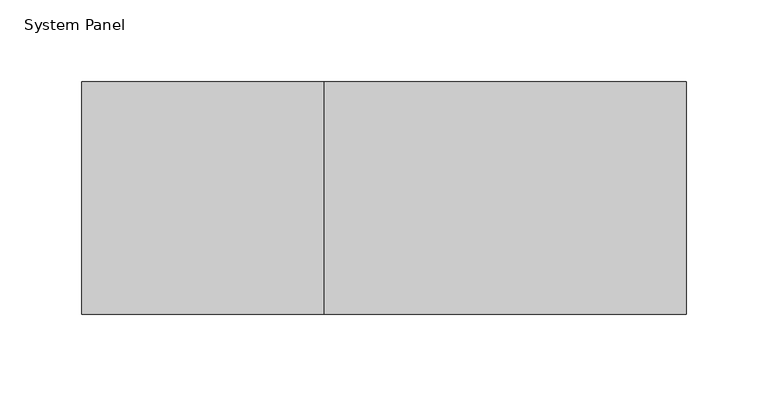
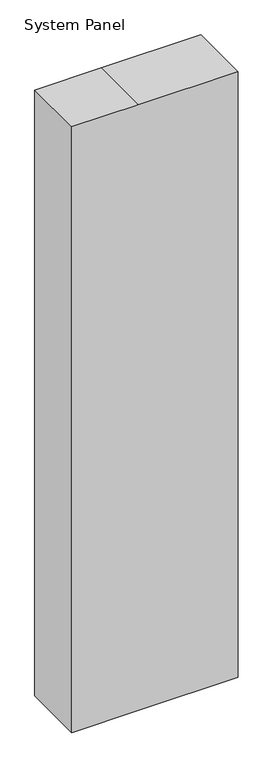
"""IFC4 building model written with IfcOpenShell, lengths in millimetres: plate geometry, System Panel : NLRS_21_CWP_hsb-vulling minerale wol 142 _gen_rsf."""

from ifc_helpers import new_model, si_unit, frame, origin, place, context, project, spatial, polyline, outline, extrude, source, transform, mapped, element, save


def system_panel_d55a1cbf(model_context):
    return source(origin(), model_context, "Body", "SweptSolid", [
        extrude(outline(polyline([(0.0, -184.5), (0.0, -36.3441061), (0.0, 184.5), (1421.0, 184.5), (1421.0, -36.3441061), (1421.0, -184.5), (0.0, -184.5)])), frame((0.0, -71.0, 0.0), z_axis=(0.0, 1.0, 0.0), x_axis=(0.0, 0.0, 1.0)), (0.0, 0.0, 1.0), 142.0),
    ])


if __name__ == "__main__":
    model = new_model("IFC4")
    model_context = context("Model", 3, world=origin())
    ifc_project = project(units=[si_unit("LENGTHUNIT", "METRE", prefix="MILLI")], contexts=[model_context])
    site = spatial("IfcSite", under=ifc_project)
    building = spatial("IfcBuilding", under=site)
    placement = place(None, origin())
    system_panel_shape = system_panel_d55a1cbf(model_context)
    element("IfcPlate", 1, ObjectType="System Panel : NLRS_21_CWP_hsb-vulling minerale wol 142 _gen_rsf", at=placement, inside=building, context=model_context, shape_type="MappedRepresentation", body=[
        mapped(system_panel_shape, transform((0.0, 0.0, 0.0), x_axis=(1.0, 0.0, 0.0), y_axis=(0.0, 1.0, 0.0), z_axis=(0.0, 0.0, 1.0))),
    ])
    save(model, "model.ifc")

# Revit data of these elements
# Type "System Panel : NLRS_21_CWP_hsb-vulling minerale wol 142 _gen_rsf"
#   Export Type to IFC As = "IfcWall"
#   Type IfcGUID = "07M7mRoiH1CR8m_RSKIwpC"
#   Assembly Code = "21.23"
# Element 1 (IfcPlate, "System Panel : NLRS_21_CWP_hsb-vulling minerale wol 142 _gen_rsf")
#   Materials on its faces: "NLRS_m1_isolatie minerale wol_gen_rsf"
# Materials
#   "NLRS_m1_isolatie minerale wol_gen_rsf": class "M - Anorganische materialen", colour RGB 200 200 140, transparency 0, Keynote = "m1", Manufacturer = "Revit Standards Foundation", URL = "www.revitstandards.org", Description = "isolatie minerale wol", Cost = 0
